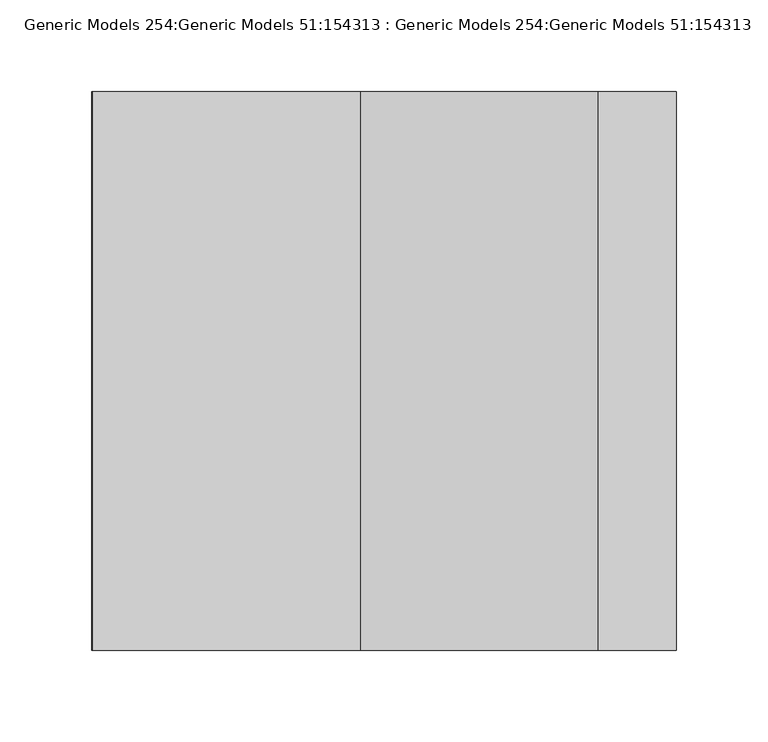
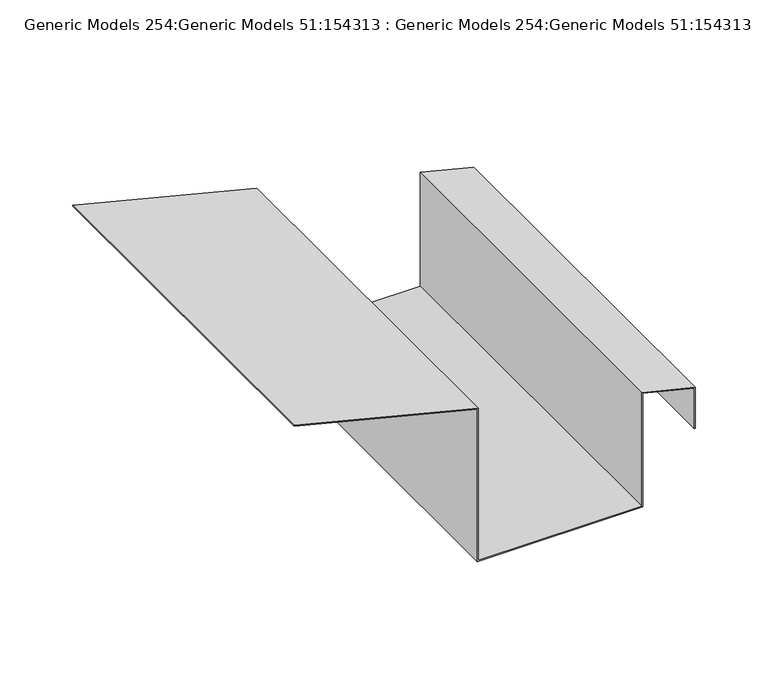
"""IFC4 building model written with IfcOpenShell, lengths in millimetres: proxy geometry, Generic Models 254:Generic Models 51:154313 : Generic Models 254:Generic Models 51:154313."""

import ifcopenshell
import ifcopenshell.guid

model = None  # the IFC model being written
_history = None  # IfcOwnerHistory: only IFC2X3 demands one
_inside = {}  # id of a spatial element -> (the spatial element, [elements in it])
_under = {}  # id of a project, library or spatial element -> (it, [spatial elements below it])
_declared = {}  # id of a project -> (the project, [libraries it declares])
_typed = {}  # id of a type object -> (the type object, [elements of that type])
_made_of = {}  # id of a material, layer set ... -> (it, [elements and type objects made of it])


def new_model(schema):
    """Start an empty IFC model of exactly this schema.

    Asked for "IFC4X3", IfcOpenShell would pick the latest addendum, in which some entities
    have other attributes; the version numbers below select the first issue.
    IFC2X3 requires an IfcOwnerHistory on every rooted entity: one is made here for all.
    """
    global model, _history
    if schema == "IFC4X3":
        model = ifcopenshell.file(schema_version=(4, 3, 0, 0))
    else:
        model = ifcopenshell.file(schema=schema)
    _inside.clear()
    _under.clear()
    _declared.clear()
    _typed.clear()
    _made_of.clear()
    _history = None
    if model.schema == "IFC2X3":
        org = make("IfcOrganization", Name="unknown")
        user = make(
            "IfcPersonAndOrganization",
            ThePerson=make("IfcPerson", FamilyName="unknown"),
            TheOrganization=org,
        )
        app = make(
            "IfcApplication",
            ApplicationDeveloper=org,
            Version="unknown",
            ApplicationFullName="unknown",
            ApplicationIdentifier="unknown",
        )
        _history = make(
            "IfcOwnerHistory",
            OwningUser=user,
            OwningApplication=app,
            ChangeAction="ADDED",
            CreationDate=0,
        )
    return model


def make(cls, **values):
    """One entity of the class cls with the attributes given. An attribute that is None is left unset."""
    return model.create_entity(
        cls, **{name: value for name, value in values.items() if value is not None}
    )


def rooted(cls, **values):
    """An entity with a GlobalId (a new one), such as an element, a storey or a relation."""
    return make(cls, GlobalId=ifcopenshell.guid.new(), OwnerHistory=_history, **values)


def si_unit(unit_type, name, prefix=None):
    """IfcSIUnit, for example si_unit("LENGTHUNIT", "METRE", prefix="MILLI")."""
    return make("IfcSIUnit", UnitType=unit_type, Prefix=prefix, Name=name)


def assignment(units):
    """IfcUnitAssignment: the units of a project."""
    return None if units is None else make("IfcUnitAssignment", Units=units)


def point(xyz):
    """IfcCartesianPoint."""
    return None if xyz is None else make("IfcCartesianPoint", Coordinates=xyz)


def direction(xyz):
    """IfcDirection."""
    return None if xyz is None else make("IfcDirection", DirectionRatios=xyz)


def frame(location, z_axis=None, x_axis=None):
    """IfcAxis2Placement3D, a coordinate frame: its origin and axes. An axis left out is left unset."""
    return make(
        "IfcAxis2Placement3D",
        Location=point(location),
        Axis=direction(z_axis),
        RefDirection=direction(x_axis),
    )


def origin():
    """The frame at (0, 0, 0) with its axes left unset."""
    return frame((0.0, 0.0, 0.0))


def place(relative_to, where):
    """IfcLocalPlacement: puts the frame where relative to a parent placement (None: the world)."""
    return make(
        "IfcLocalPlacement", PlacementRelTo=relative_to, RelativePlacement=where
    )


def context(
    kind, dimensions, precision=None, world=None, true_north=None, identifier=None
):
    """IfcGeometricRepresentationContext, for example the 3D "Model" context."""
    return make(
        "IfcGeometricRepresentationContext",
        ContextIdentifier=identifier,
        ContextType=kind,
        CoordinateSpaceDimension=dimensions,
        Precision=precision,
        WorldCoordinateSystem=world,
        TrueNorth=true_north,
    )


def project(units=None, contexts=None):
    """IfcProject with its units and contexts."""
    return rooted(
        "IfcProject",
        Name="project",
        RepresentationContexts=contexts,
        UnitsInContext=assignment(units),
    )


def spatial(cls, under=None, at=None, **own):
    """A site, building, storey or space (cls), placed at a placement, below another one or the project."""
    s = rooted(cls, ObjectPlacement=at, **own)
    if under is not None:
        _under.setdefault(under.id(), (under, []))[1].append(s)
    return s


def polyline(points):
    """IfcPolyline through the points."""
    return make("IfcPolyline", Points=[point(p) for p in points])


def outline(outer, holes=None, kind="AREA"):
    """IfcArbitraryClosedProfileDef: a profile drawn as a closed curve; with holes, ...WithVoids."""
    if holes is None:
        return make("IfcArbitraryClosedProfileDef", ProfileType=kind, OuterCurve=outer)
    return make(
        "IfcArbitraryProfileDefWithVoids",
        ProfileType=kind,
        OuterCurve=outer,
        InnerCurves=holes,
    )


def extrude(swept, where, along, depth):
    """IfcExtrudedAreaSolid: the profile swept, set in the frame where, extruded along a direction by depth."""
    return make(
        "IfcExtrudedAreaSolid",
        SweptArea=swept,
        Position=where,
        ExtrudedDirection=direction(along),
        Depth=depth,
    )


def shape(context_of_items, identifier, shape_type, items):
    """IfcShapeRepresentation: the items that make up one representation, for example the "Body"."""
    return make(
        "IfcShapeRepresentation",
        ContextOfItems=context_of_items,
        RepresentationIdentifier=identifier,
        RepresentationType=shape_type,
        Items=items,
    )


def source(mapping_origin, context_of_items, identifier, shape_type, items):
    """IfcRepresentationMap: a shape defined once, which mapped items show again and again."""
    return make(
        "IfcRepresentationMap",
        MappingOrigin=mapping_origin,
        MappedRepresentation=shape(context_of_items, identifier, shape_type, items),
    )


def transform(
    local_origin,
    x_axis=None,
    y_axis=None,
    z_axis=None,
    scale=None,
    scale2=None,
    scale3=None,
    uniform=True,
):
    """IfcCartesianTransformationOperator3D, or its non-uniform kind. x_axis, y_axis, z_axis: its Axis1, 2, 3."""
    if uniform:
        return make(
            "IfcCartesianTransformationOperator3D",
            Axis1=direction(x_axis),
            Axis2=direction(y_axis),
            LocalOrigin=point(local_origin),
            Scale=scale,
            Axis3=direction(z_axis),
        )
    return make(
        "IfcCartesianTransformationOperator3DnonUniform",
        Axis1=direction(x_axis),
        Axis2=direction(y_axis),
        LocalOrigin=point(local_origin),
        Scale=scale,
        Axis3=direction(z_axis),
        Scale2=scale2,
        Scale3=scale3,
    )


def mapped(mapping_source, mapping_target):
    """IfcMappedItem: shows the shape of a source again, moved by a transform."""
    return make(
        "IfcMappedItem", MappingSource=mapping_source, MappingTarget=mapping_target
    )


def made_of(thing, what):
    """Note that an element or type object is made of a material, layer set ...; save() writes the relation."""
    if what is not None:
        _made_of.setdefault(what.id(), (what, []))[1].append(thing)
    return thing


def element(
    cls,
    number,
    at=None,
    inside=None,
    cuts=None,
    type_object=None,
    material=None,
    context=None,
    identifier="Body",
    shape_type=None,
    held_by="IfcProductDefinitionShape",
    body=None,
    shapes=None,
    **own,
):
    """One element of the class cls, such as IfcWall. Its Tag is "e" and its number.

    at: its placement. inside: the storey or other place that contains it. cuts: it is an
    opening in that element (IfcRelVoidsElement). A single representation is given by context,
    identifier, shape_type and body (its items); several are given by shapes. held_by: the class
    of the entity that holds the representations. save() writes the other relations.
    """
    e = rooted(cls, Tag="e%d" % number, ObjectPlacement=at, **own)
    if body is not None:
        shapes = [shape(context, identifier, shape_type, body)]
    if shapes is not None:
        e.Representation = make(held_by, Representations=shapes)
    if inside is not None:
        _inside.setdefault(inside.id(), (inside, []))[1].append(e)
    if cuts is not None:
        rooted(
            "IfcRelVoidsElement", RelatingBuildingElement=cuts, RelatedOpeningElement=e
        )
    if type_object is not None:
        _typed.setdefault(type_object.id(), (type_object, []))[1].append(e)
    return made_of(e, material)


def aggregate(whole, parts):
    """IfcRelAggregates: a whole, such as a stair, and the parts it consists of."""
    return rooted("IfcRelAggregates", RelatingObject=whole, RelatedObjects=parts)


def save(model, path):
    """Write the relations noted so far, then the file.

    IfcRelAggregates (storeys below a building ...), IfcRelContainedInSpatialStructure (elements
    in a storey), IfcRelDefinesByType, IfcRelAssociatesMaterial and IfcRelDeclares: one each for
    every whole, place, type object, material and project.
    """
    for whole, parts in _under.values():
        aggregate(whole, parts)
    for where, things in _inside.values():
        rooted(
            "IfcRelContainedInSpatialStructure",
            RelatedElements=things,
            RelatingStructure=where,
        )
    for kind, things in _typed.values():
        rooted("IfcRelDefinesByType", RelatedObjects=things, RelatingType=kind)
    for what, things in _made_of.values():
        rooted("IfcRelAssociatesMaterial", RelatedObjects=things, RelatingMaterial=what)
    for by, libraries in _declared.values():
        rooted("IfcRelDeclares", RelatingContext=by, RelatedDefinitions=libraries)
    model.write(path)


def generic_models_254_generic_models_51_154313_generic_models_ec08a3f1(model_context):
    return source(origin(), model_context, "Body", "SweptSolid", [
        extrude(outline(polyline([(6454.4396974, 1764.50351), (6418.051444, 1910.0565238), (6290.0265264, 1910.0565238), (6290.0265264, 2041.403213), (6385.2765264, 2041.403213), (6375.0255938, 2082.5174582), (6341.3699291, 2082.5174582), (6341.3699291, 2083.3112082), (6375.6457393, 2083.3112082), (6386.2924801, 2040.609463), (6290.8202764, 2040.609463), (6290.8202764, 1910.8502738), (6418.6711852, 1910.8502738), (6455.209748, 1764.6960227), (6454.4396974, 1764.50351)])), frame((0.0, 5312.3878092, 0.0), z_axis=(0.0, 1.0, 0.0), x_axis=(0.0, 0.0, 1.0)), (0.0, 0.0, 1.0), 304.8),
    ])


if __name__ == "__main__":
    model = new_model("IFC4")
    model_context = context("Model", 3, world=origin())
    ifc_project = project(units=[si_unit("LENGTHUNIT", "METRE", prefix="MILLI")], contexts=[model_context])
    site = spatial("IfcSite", under=ifc_project)
    building = spatial("IfcBuilding", under=site)
    placement = place(None, origin())
    generic_models_254_generic_models_51_154313_generic_models_shape = generic_models_254_generic_models_51_154313_generic_models_ec08a3f1(model_context)
    element("IfcBuildingElementProxy", 1, Name="Generic Models 254:Generic Models 51:154313 : Generic Models 254:Generic Models 51:154313", ObjectType="Generic Models 254:Generic Models 51:154313 : Generic Models 254:Generic Models 51:154313", at=placement, inside=building, context=model_context, shape_type="MappedRepresentation", body=[
        mapped(generic_models_254_generic_models_51_154313_generic_models_shape, transform((0.0, 0.0, 0.0), x_axis=(1.0, 0.0, 0.0), y_axis=(0.0, 1.0, 0.0), z_axis=(0.0, 0.0, 1.0))),
    ])
    save(model, "model.ifc")

# Revit data of these elements
# Type "Generic Models 254:Generic Models 51:154313 : Generic Models 254:Generic Models 51:154313"
#   NameOverride = "Generic Models 254:Generic Models 51:154313"
#   ObjectTypeOverride = "Generic Models 254:Generic Models 51"
#   Reference = "Generic Models 51"
#   Category = "Generic Models"
#   Tag = "154313"
# Element 1 (IfcBuildingElementProxy, "Generic Models 254:Generic Models 51:154313 : Generic Models 254:Generic Models 51:154313")
#   Materials on its faces: "_SELF ADHERED MEMBRANE 21796"
# Materials
#   "_SELF ADHERED MEMBRANE 21796": class "Unassigned", colour RGB 253 192 103, transparency 0
